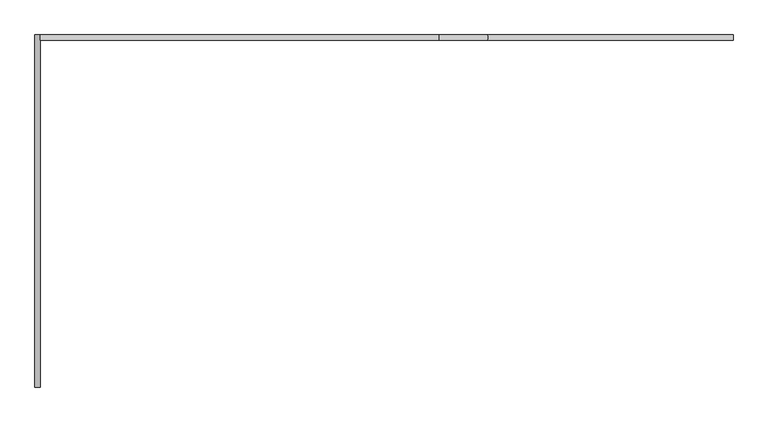
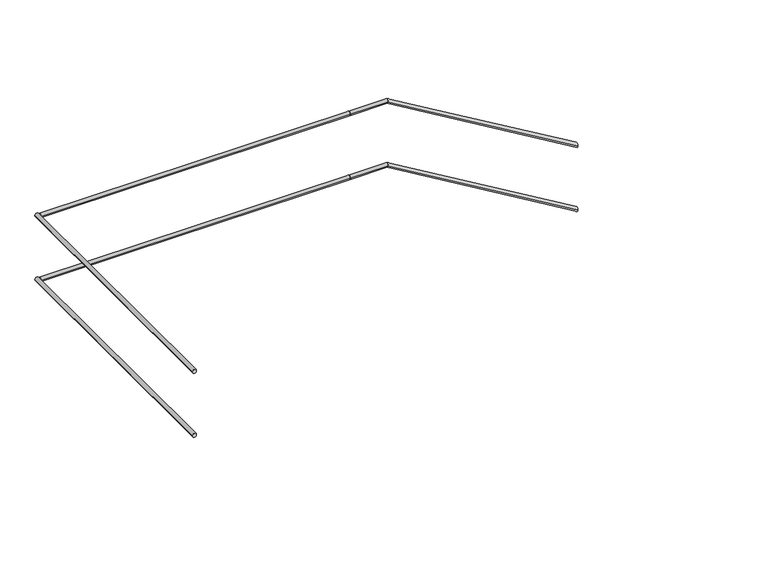
"""IFC4 building model written with IfcOpenShell, lengths in millimetres: railing geometry."""

import ifcopenshell
import ifcopenshell.guid

model = None  # the IFC model being written
_history = None  # IfcOwnerHistory: only IFC2X3 demands one
_inside = {}  # id of a spatial element -> (the spatial element, [elements in it])
_under = {}  # id of a project, library or spatial element -> (it, [spatial elements below it])
_declared = {}  # id of a project -> (the project, [libraries it declares])
_typed = {}  # id of a type object -> (the type object, [elements of that type])
_made_of = {}  # id of a material, layer set ... -> (it, [elements and type objects made of it])


def new_model(schema):
    """Start an empty IFC model of exactly this schema.

    Asked for "IFC4X3", IfcOpenShell would pick the latest addendum, in which some entities
    have other attributes; the version numbers below select the first issue.
    IFC2X3 requires an IfcOwnerHistory on every rooted entity: one is made here for all.
    """
    global model, _history
    if schema == "IFC4X3":
        model = ifcopenshell.file(schema_version=(4, 3, 0, 0))
    else:
        model = ifcopenshell.file(schema=schema)
    _inside.clear()
    _under.clear()
    _declared.clear()
    _typed.clear()
    _made_of.clear()
    _history = None
    if model.schema == "IFC2X3":
        org = make("IfcOrganization", Name="unknown")
        user = make(
            "IfcPersonAndOrganization",
            ThePerson=make("IfcPerson", FamilyName="unknown"),
            TheOrganization=org,
        )
        app = make(
            "IfcApplication",
            ApplicationDeveloper=org,
            Version="unknown",
            ApplicationFullName="unknown",
            ApplicationIdentifier="unknown",
        )
        _history = make(
            "IfcOwnerHistory",
            OwningUser=user,
            OwningApplication=app,
            ChangeAction="ADDED",
            CreationDate=0,
        )
    return model


def make(cls, **values):
    """One entity of the class cls with the attributes given. An attribute that is None is left unset."""
    return model.create_entity(
        cls, **{name: value for name, value in values.items() if value is not None}
    )


def rooted(cls, **values):
    """An entity with a GlobalId (a new one), such as an element, a storey or a relation."""
    return make(cls, GlobalId=ifcopenshell.guid.new(), OwnerHistory=_history, **values)


def si_unit(unit_type, name, prefix=None):
    """IfcSIUnit, for example si_unit("LENGTHUNIT", "METRE", prefix="MILLI")."""
    return make("IfcSIUnit", UnitType=unit_type, Prefix=prefix, Name=name)


def assignment(units):
    """IfcUnitAssignment: the units of a project."""
    return None if units is None else make("IfcUnitAssignment", Units=units)


def point(xyz):
    """IfcCartesianPoint."""
    return None if xyz is None else make("IfcCartesianPoint", Coordinates=xyz)


def direction(xyz):
    """IfcDirection."""
    return None if xyz is None else make("IfcDirection", DirectionRatios=xyz)


def frame(location, z_axis=None, x_axis=None):
    """IfcAxis2Placement3D, a coordinate frame: its origin and axes. An axis left out is left unset."""
    return make(
        "IfcAxis2Placement3D",
        Location=point(location),
        Axis=direction(z_axis),
        RefDirection=direction(x_axis),
    )


def origin():
    """The frame at (0, 0, 0) with its axes left unset."""
    return frame((0.0, 0.0, 0.0))


def place(relative_to, where):
    """IfcLocalPlacement: puts the frame where relative to a parent placement (None: the world)."""
    return make(
        "IfcLocalPlacement", PlacementRelTo=relative_to, RelativePlacement=where
    )


def context(
    kind, dimensions, precision=None, world=None, true_north=None, identifier=None
):
    """IfcGeometricRepresentationContext, for example the 3D "Model" context."""
    return make(
        "IfcGeometricRepresentationContext",
        ContextIdentifier=identifier,
        ContextType=kind,
        CoordinateSpaceDimension=dimensions,
        Precision=precision,
        WorldCoordinateSystem=world,
        TrueNorth=true_north,
    )


def project(units=None, contexts=None):
    """IfcProject with its units and contexts."""
    return rooted(
        "IfcProject",
        Name="project",
        RepresentationContexts=contexts,
        UnitsInContext=assignment(units),
    )


def spatial(cls, under=None, at=None, **own):
    """A site, building, storey or space (cls), placed at a placement, below another one or the project."""
    s = rooted(cls, ObjectPlacement=at, **own)
    if under is not None:
        _under.setdefault(under.id(), (under, []))[1].append(s)
    return s


def circle_curve(where, radius):
    """IfcCircle in the frame where."""
    return make("IfcCircle", Position=where, Radius=radius)


def ellipse_curve(where, semi_axis1, semi_axis2):
    """IfcEllipse in the frame where."""
    return make(
        "IfcEllipse", Position=where, SemiAxis1=semi_axis1, SemiAxis2=semi_axis2
    )


def shape(context_of_items, identifier, shape_type, items):
    """IfcShapeRepresentation: the items that make up one representation, for example the "Body"."""
    return make(
        "IfcShapeRepresentation",
        ContextOfItems=context_of_items,
        RepresentationIdentifier=identifier,
        RepresentationType=shape_type,
        Items=items,
    )


def source(mapping_origin, context_of_items, identifier, shape_type, items):
    """IfcRepresentationMap: a shape defined once, which mapped items show again and again."""
    return make(
        "IfcRepresentationMap",
        MappingOrigin=mapping_origin,
        MappedRepresentation=shape(context_of_items, identifier, shape_type, items),
    )


def transform(
    local_origin,
    x_axis=None,
    y_axis=None,
    z_axis=None,
    scale=None,
    scale2=None,
    scale3=None,
    uniform=True,
):
    """IfcCartesianTransformationOperator3D, or its non-uniform kind. x_axis, y_axis, z_axis: its Axis1, 2, 3."""
    if uniform:
        return make(
            "IfcCartesianTransformationOperator3D",
            Axis1=direction(x_axis),
            Axis2=direction(y_axis),
            LocalOrigin=point(local_origin),
            Scale=scale,
            Axis3=direction(z_axis),
        )
    return make(
        "IfcCartesianTransformationOperator3DnonUniform",
        Axis1=direction(x_axis),
        Axis2=direction(y_axis),
        LocalOrigin=point(local_origin),
        Scale=scale,
        Axis3=direction(z_axis),
        Scale2=scale2,
        Scale3=scale3,
    )


def mapped(mapping_source, mapping_target):
    """IfcMappedItem: shows the shape of a source again, moved by a transform."""
    return make(
        "IfcMappedItem", MappingSource=mapping_source, MappingTarget=mapping_target
    )


def made_of(thing, what):
    """Note that an element or type object is made of a material, layer set ...; save() writes the relation."""
    if what is not None:
        _made_of.setdefault(what.id(), (what, []))[1].append(thing)
    return thing


def element(
    cls,
    number,
    at=None,
    inside=None,
    cuts=None,
    type_object=None,
    material=None,
    context=None,
    identifier="Body",
    shape_type=None,
    held_by="IfcProductDefinitionShape",
    body=None,
    shapes=None,
    **own,
):
    """One element of the class cls, such as IfcWall. Its Tag is "e" and its number.

    at: its placement. inside: the storey or other place that contains it. cuts: it is an
    opening in that element (IfcRelVoidsElement). A single representation is given by context,
    identifier, shape_type and body (its items); several are given by shapes. held_by: the class
    of the entity that holds the representations. save() writes the other relations.
    """
    e = rooted(cls, Tag="e%d" % number, ObjectPlacement=at, **own)
    if body is not None:
        shapes = [shape(context, identifier, shape_type, body)]
    if shapes is not None:
        e.Representation = make(held_by, Representations=shapes)
    if inside is not None:
        _inside.setdefault(inside.id(), (inside, []))[1].append(e)
    if cuts is not None:
        rooted(
            "IfcRelVoidsElement", RelatingBuildingElement=cuts, RelatedOpeningElement=e
        )
    if type_object is not None:
        _typed.setdefault(type_object.id(), (type_object, []))[1].append(e)
    return made_of(e, material)


def aggregate(whole, parts):
    """IfcRelAggregates: a whole, such as a stair, and the parts it consists of."""
    return rooted("IfcRelAggregates", RelatingObject=whole, RelatedObjects=parts)


def save(model, path):
    """Write the relations noted so far, then the file.

    IfcRelAggregates (storeys below a building ...), IfcRelContainedInSpatialStructure (elements
    in a storey), IfcRelDefinesByType, IfcRelAssociatesMaterial and IfcRelDeclares: one each for
    every whole, place, type object, material and project.
    """
    for whole, parts in _under.values():
        aggregate(whole, parts)
    for where, things in _inside.values():
        rooted(
            "IfcRelContainedInSpatialStructure",
            RelatedElements=things,
            RelatingStructure=where,
        )
    for kind, things in _typed.values():
        rooted("IfcRelDefinesByType", RelatedObjects=things, RelatingType=kind)
    for what, things in _made_of.values():
        rooted("IfcRelAssociatesMaterial", RelatedObjects=things, RelatingMaterial=what)
    for by, libraries in _declared.values():
        rooted("IfcRelDeclares", RelatingContext=by, RelatedDefinitions=libraries)
    model.write(path)


def plane_surface(at):
    """IfcPlane: the flat surface through the origin of the frame at, square to its z axis."""
    return make("IfcPlane", Position=at)


def cylinder_surface(at, radius):
    """IfcCylindricalSurface: all points at the distance radius from the z axis of the frame at."""
    return make("IfcCylindricalSurface", Position=at, Radius=radius)


def advanced_brep(points, edges, surfaces, faces):
    """IfcAdvancedBrep: a solid bounded by faces that lie on surfaces and meet in shared edges.

    An edge is (start, end): straight between two places in points (the first is 0);
    or (start, end, curve); or (start, end, curve, False) where it runs against its curve.
    A face is (place in surfaces, loops), or (place, loops, False) where it looks against
    its surface's normal. A loop lists edges by number (the first is 1), with a minus sign
    where the edge is run from its end to its start. The first loop is the outer one.
    """
    corners = [point(p) for p in points]
    vertices = [make("IfcVertexPoint", VertexGeometry=c) for c in corners]
    made = []
    for start, end, *more in edges:
        made.append(
            make(
                "IfcEdgeCurve",
                EdgeStart=vertices[start],
                EdgeEnd=vertices[end],
                EdgeGeometry=more[0] if more else make("IfcPolyline", Points=[corners[start], corners[end]]),
                SameSense=more[1] if len(more) > 1 else True,
            )
        )
    hull = []
    for where, loops, *sense in faces:
        bounds = []
        for j, loop in enumerate(loops):
            ring = [make("IfcOrientedEdge", EdgeElement=made[abs(k) - 1], Orientation=k > 0) for k in loop]
            bounds.append(
                make(
                    "IfcFaceOuterBound" if j == 0 else "IfcFaceBound",
                    Bound=make("IfcEdgeLoop", EdgeList=ring),
                    Orientation=True,
                )
            )
        hull.append(make("IfcAdvancedFace", Bounds=bounds, FaceSurface=surfaces[where], SameSense=sense[0] if sense else True))
    return make("IfcAdvancedBrep", Outer=make("IfcClosedShell", CfsFaces=hull))


def railing_74e482c1(model_context):
    return source(origin(), model_context, "Body", "AdvancedBrep", [
        advanced_brep(
        [(33043.8956602, 25734.1208589, 899.1723166), (33043.8956602, 25764.1208589, 899.1723166), (31639.7692216, 25734.1208589, 1734.9618634), (31639.7692216, 25764.1208589, 1734.9618634), (31363.8956602, 25734.1208589, 1734.9618634), (31363.8956602, 25764.1208589, 1734.9618634)],
        [
            (0, 1, ellipse_curve(frame((33043.8956602, 25749.1208589, 899.1723166), z_axis=(1.0, 0.0, 0.0), x_axis=(0.0, 0.0, -1.0)), 17.4562134, 15.0)),
            (1, 0, ellipse_curve(frame((33043.8956602, 25749.1208589, 899.1723166), z_axis=(1.0, 0.0, 0.0), x_axis=(0.0, 0.0, -1.0)), 17.4562134, 15.0)),
            (0, 2),
            (2, 3, ellipse_curve(frame((31639.7692216, 25749.1208589, 1734.9618634), z_axis=(0.9641817474962142, 0.0, -0.26524245096731175), x_axis=(-0.26524245096731197, 0.0, -0.964181747496214)), 15.5572329, 15.0)),
            (3, 1),
            (3, 2, ellipse_curve(frame((31639.7692216, 25749.1208589, 1734.9618634), z_axis=(0.9641817474962142, 0.0, -0.26524245096731175), x_axis=(-0.26524245096731197, 0.0, -0.964181747496214)), 15.5572329, 15.0)),
            (4, 5, circle_curve(frame((31363.8956602, 25749.1208589, 1734.9618634), z_axis=(-1.0, 0.0, 0.0), x_axis=(0.0, 1.0, 0.0)), 15.0)),
            (5, 4, circle_curve(frame((31363.8956602, 25749.1208589, 1734.9618634), z_axis=(-1.0, 0.0, 0.0), x_axis=(0.0, 1.0, 0.0)), 15.0)),
            (2, 4),
            (5, 3),
        ],
        [
            plane_surface(frame((33043.8956602, 25749.1208589, 916.62853), z_axis=(1.0, 0.0, 0.0), x_axis=(0.0, -1.0, 0.0))),
            cylinder_surface(frame((33036.2234023, 25749.1208589, 903.7391368), z_axis=(0.8592928844097065, 0.0, -0.5114838597676831), x_axis=(0.0, 1.0, 0.0)), 15.0),
            plane_surface(frame((31363.8956602, 25749.1208589, 1749.9618634), z_axis=(-1.0, 0.0, 0.0), x_axis=(0.0, -1.0, 0.0))),
            cylinder_surface(frame((31643.8956602, 25749.1208589, 1734.9618634), z_axis=(1.0, 0.0, 0.0), x_axis=(0.0, 1.0, 0.0)), 15.0),
        ],
        [
            (0, [[1, 2]]),
            (1, [[-1, 3, 4, 5]]),
            (1, [[-2, -5, 6, -3]]),
            (2, [[7, 8]]),
            (3, [[-4, 9, -8, 10]]),
            (3, [[-6, -10, -7, -9]]),
        ],
    ),
        advanced_brep(
        [(31363.8956602, 25734.1208589, 1734.9618634), (31363.8956602, 25764.1208589, 1734.9618634), (29079.2956602, 25734.1208589, 1734.9618634), (29079.2956602, 25764.1208589, 1734.9618634)],
        [
            (0, 1, circle_curve(frame((31363.8956602, 25749.1208589, 1734.9618634), z_axis=(1.0, 0.0, 0.0), x_axis=(0.0, 1.0, 0.0)), 15.0)),
            (1, 0, circle_curve(frame((31363.8956602, 25749.1208589, 1734.9618634), z_axis=(1.0, 0.0, 0.0), x_axis=(0.0, 1.0, 0.0)), 15.0)),
            (2, 3, circle_curve(frame((29079.2956602, 25749.1208589, 1734.9618634), z_axis=(-1.0, 0.0, 0.0), x_axis=(0.0, 1.0, 0.0)), 15.0)),
            (3, 2, circle_curve(frame((29079.2956602, 25749.1208589, 1734.9618634), z_axis=(-1.0, 0.0, 0.0), x_axis=(0.0, 1.0, 0.0)), 15.0)),
            (0, 2),
            (3, 1),
        ],
        [
            plane_surface(frame((31363.8956602, 25749.1208589, 1749.9618634), z_axis=(1.0, 0.0, 0.0), x_axis=(0.0, -1.0, 0.0))),
            plane_surface(frame((29079.2956602, 25749.1208589, 1749.9618634), z_axis=(-1.0, 0.0, 0.0), x_axis=(0.0, -1.0, 0.0))),
            cylinder_surface(frame((31363.8956602, 25749.1208589, 1734.9618634), z_axis=(1.0, 0.0, 0.0), x_axis=(0.0, 1.0, 0.0)), 15.0),
        ],
        [
            (0, [[1, 2]]),
            (1, [[3, 4]]),
            (2, [[-1, 5, -4, 6]]),
            (2, [[-2, -6, -3, -5]]),
        ],
    ),
        advanced_brep(
        [(29079.2956602, 25764.1208589, 1734.9618634), (29049.2956602, 25764.1208589, 1734.9618634), (29079.2956602, 23749.5208589, 1734.9618634), (29049.2956602, 23749.5208589, 1734.9618634)],
        [
            (0, 1, circle_curve(frame((29064.2956602, 25764.1208589, 1734.9618634), z_axis=(0.0, 1.0, 0.0), x_axis=(-1.0, 0.0, 0.0)), 15.0)),
            (1, 0, circle_curve(frame((29064.2956602, 25764.1208589, 1734.9618634), z_axis=(0.0, 1.0, 0.0), x_axis=(-1.0, 0.0, 0.0)), 15.0)),
            (2, 3, circle_curve(frame((29064.2956602, 23749.5208589, 1734.9618634), z_axis=(0.0, -1.0, 0.0), x_axis=(-1.0, 0.0, 0.0)), 15.0)),
            (3, 2, circle_curve(frame((29064.2956602, 23749.5208589, 1734.9618634), z_axis=(0.0, -1.0, 0.0), x_axis=(-1.0, 0.0, 0.0)), 15.0)),
            (0, 2),
            (3, 1),
        ],
        [
            plane_surface(frame((29064.2956602, 25764.1208589, 1749.9618634), z_axis=(0.0, 1.0, 0.0), x_axis=(0.0, 0.0, -1.0))),
            plane_surface(frame((29064.2956602, 23749.5208589, 1749.9618634), z_axis=(0.0, -1.0, 0.0), x_axis=(0.0, 0.0, -1.0))),
            cylinder_surface(frame((29064.2956602, 25764.1208589, 1734.9618634), z_axis=(0.0, 1.0, 0.0), x_axis=(-1.0, 0.0, 0.0)), 15.0),
        ],
        [
            (0, [[1, 2]]),
            (1, [[3, 4]]),
            (2, [[-1, 5, -4, 6]]),
            (2, [[-2, -6, -3, -5]]),
        ],
    ),
        advanced_brep(
        [(33043.8956602, 25734.1208589, 1399.1723166), (33043.8956602, 25764.1208589, 1399.1723166), (31639.7692216, 25734.1208589, 2234.9618634), (31639.7692216, 25764.1208589, 2234.9618634), (31363.8956602, 25734.1208589, 2234.9618634), (31363.8956602, 25764.1208589, 2234.9618634)],
        [
            (0, 1, ellipse_curve(frame((33043.8956602, 25749.1208589, 1399.1723166), z_axis=(1.0, 0.0, 0.0), x_axis=(0.0, 0.0, -1.0)), 17.4562134, 15.0)),
            (1, 0, ellipse_curve(frame((33043.8956602, 25749.1208589, 1399.1723166), z_axis=(1.0, 0.0, 0.0), x_axis=(0.0, 0.0, -1.0)), 17.4562134, 15.0)),
            (0, 2),
            (2, 3, ellipse_curve(frame((31639.7692216, 25749.1208589, 2234.9618634), z_axis=(0.9641817474962142, 0.0, -0.26524245096731175), x_axis=(-0.26524245096731197, 0.0, -0.964181747496214)), 15.5572329, 15.0)),
            (3, 1),
            (3, 2, ellipse_curve(frame((31639.7692216, 25749.1208589, 2234.9618634), z_axis=(0.9641817474962142, 0.0, -0.26524245096731175), x_axis=(-0.26524245096731197, 0.0, -0.964181747496214)), 15.5572329, 15.0)),
            (4, 5, circle_curve(frame((31363.8956602, 25749.1208589, 2234.9618634), z_axis=(-1.0, 0.0, 0.0), x_axis=(0.0, 1.0, 0.0)), 15.0)),
            (5, 4, circle_curve(frame((31363.8956602, 25749.1208589, 2234.9618634), z_axis=(-1.0, 0.0, 0.0), x_axis=(0.0, 1.0, 0.0)), 15.0)),
            (2, 4),
            (5, 3),
        ],
        [
            plane_surface(frame((33043.8956602, 25749.1208589, 1416.62853), z_axis=(1.0, 0.0, 0.0), x_axis=(0.0, -1.0, 0.0))),
            cylinder_surface(frame((33036.2234023, 25749.1208589, 1403.7391368), z_axis=(0.8592928844097065, 0.0, -0.5114838597676831), x_axis=(0.0, 1.0, 0.0)), 15.0),
            plane_surface(frame((31363.8956602, 25749.1208589, 2249.9618634), z_axis=(-1.0, 0.0, 0.0), x_axis=(0.0, -1.0, 0.0))),
            cylinder_surface(frame((31643.8956602, 25749.1208589, 2234.9618634), z_axis=(1.0, 0.0, 0.0), x_axis=(0.0, 1.0, 0.0)), 15.0),
        ],
        [
            (0, [[1, 2]]),
            (1, [[-1, 3, 4, 5]]),
            (1, [[-2, -5, 6, -3]]),
            (2, [[7, 8]]),
            (3, [[-4, 9, -8, 10]]),
            (3, [[-6, -10, -7, -9]]),
        ],
    ),
        advanced_brep(
        [(31363.8956602, 25734.1208589, 2234.9618634), (31363.8956602, 25764.1208589, 2234.9618634), (29079.2956602, 25734.1208589, 2234.9618634), (29079.2956602, 25764.1208589, 2234.9618634)],
        [
            (0, 1, circle_curve(frame((31363.8956602, 25749.1208589, 2234.9618634), z_axis=(1.0, 0.0, 0.0), x_axis=(0.0, 1.0, 0.0)), 15.0)),
            (1, 0, circle_curve(frame((31363.8956602, 25749.1208589, 2234.9618634), z_axis=(1.0, 0.0, 0.0), x_axis=(0.0, 1.0, 0.0)), 15.0)),
            (2, 3, circle_curve(frame((29079.2956602, 25749.1208589, 2234.9618634), z_axis=(-1.0, 0.0, 0.0), x_axis=(0.0, 1.0, 0.0)), 15.0)),
            (3, 2, circle_curve(frame((29079.2956602, 25749.1208589, 2234.9618634), z_axis=(-1.0, 0.0, 0.0), x_axis=(0.0, 1.0, 0.0)), 15.0)),
            (0, 2),
            (3, 1),
        ],
        [
            plane_surface(frame((31363.8956602, 25749.1208589, 2249.9618634), z_axis=(1.0, 0.0, 0.0), x_axis=(0.0, -1.0, 0.0))),
            plane_surface(frame((29079.2956602, 25749.1208589, 2249.9618634), z_axis=(-1.0, 0.0, 0.0), x_axis=(0.0, -1.0, 0.0))),
            cylinder_surface(frame((31363.8956602, 25749.1208589, 2234.9618634), z_axis=(1.0, 0.0, 0.0), x_axis=(0.0, 1.0, 0.0)), 15.0),
        ],
        [
            (0, [[1, 2]]),
            (1, [[3, 4]]),
            (2, [[-1, 5, -4, 6]]),
            (2, [[-2, -6, -3, -5]]),
        ],
    ),
        advanced_brep(
        [(29079.2956602, 25764.1208589, 2234.9618634), (29049.2956602, 25764.1208589, 2234.9618634), (29079.2956602, 23749.5208589, 2234.9618634), (29049.2956602, 23749.5208589, 2234.9618634)],
        [
            (0, 1, circle_curve(frame((29064.2956602, 25764.1208589, 2234.9618634), z_axis=(0.0, 1.0, 0.0), x_axis=(-1.0, 0.0, 0.0)), 15.0)),
            (1, 0, circle_curve(frame((29064.2956602, 25764.1208589, 2234.9618634), z_axis=(0.0, 1.0, 0.0), x_axis=(-1.0, 0.0, 0.0)), 15.0)),
            (2, 3, circle_curve(frame((29064.2956602, 23749.5208589, 2234.9618634), z_axis=(0.0, -1.0, 0.0), x_axis=(-1.0, 0.0, 0.0)), 15.0)),
            (3, 2, circle_curve(frame((29064.2956602, 23749.5208589, 2234.9618634), z_axis=(0.0, -1.0, 0.0), x_axis=(-1.0, 0.0, 0.0)), 15.0)),
            (0, 2),
            (3, 1),
        ],
        [
            plane_surface(frame((29064.2956602, 25764.1208589, 2249.9618634), z_axis=(0.0, 1.0, 0.0), x_axis=(0.0, 0.0, -1.0))),
            plane_surface(frame((29064.2956602, 23749.5208589, 2249.9618634), z_axis=(0.0, -1.0, 0.0), x_axis=(0.0, 0.0, -1.0))),
            cylinder_surface(frame((29064.2956602, 25764.1208589, 2234.9618634), z_axis=(0.0, 1.0, 0.0), x_axis=(-1.0, 0.0, 0.0)), 15.0),
        ],
        [
            (0, [[1, 2]]),
            (1, [[3, 4]]),
            (2, [[-1, 5, -4, 6]]),
            (2, [[-2, -6, -3, -5]]),
        ],
    ),
    ])


if __name__ == "__main__":
    model = new_model("IFC4")
    model_context = context("Model", 3, world=origin())
    ifc_project = project(units=[si_unit("LENGTHUNIT", "METRE", prefix="MILLI")], contexts=[model_context])
    site = spatial("IfcSite", under=ifc_project)
    building = spatial("IfcBuilding", under=site)
    placement = place(None, origin())
    railing_shape = railing_74e482c1(model_context)
    element("IfcRailing", 1, at=placement, inside=building, context=model_context, shape_type="MappedRepresentation", body=[
        mapped(railing_shape, transform((0.0, 0.0, 0.0), x_axis=(1.0, 0.0, 0.0), y_axis=(0.0, 1.0, 0.0), z_axis=(0.0, 0.0, 1.0))),
    ])
    save(model, "model.ifc")
